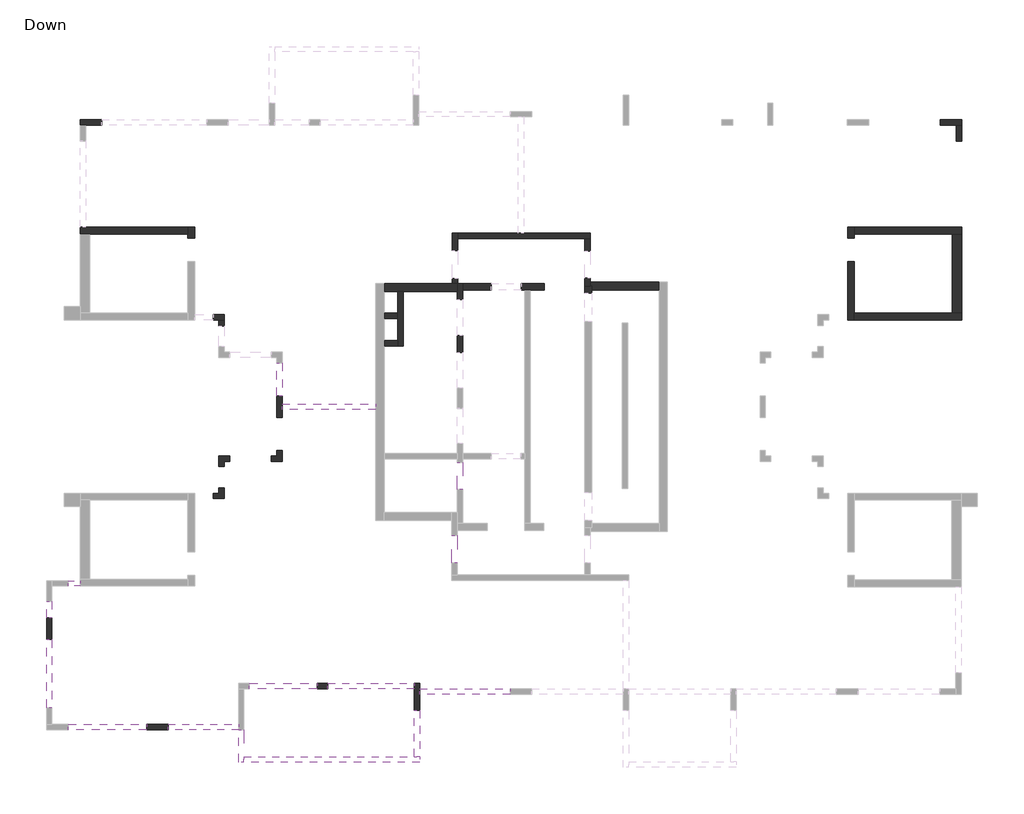
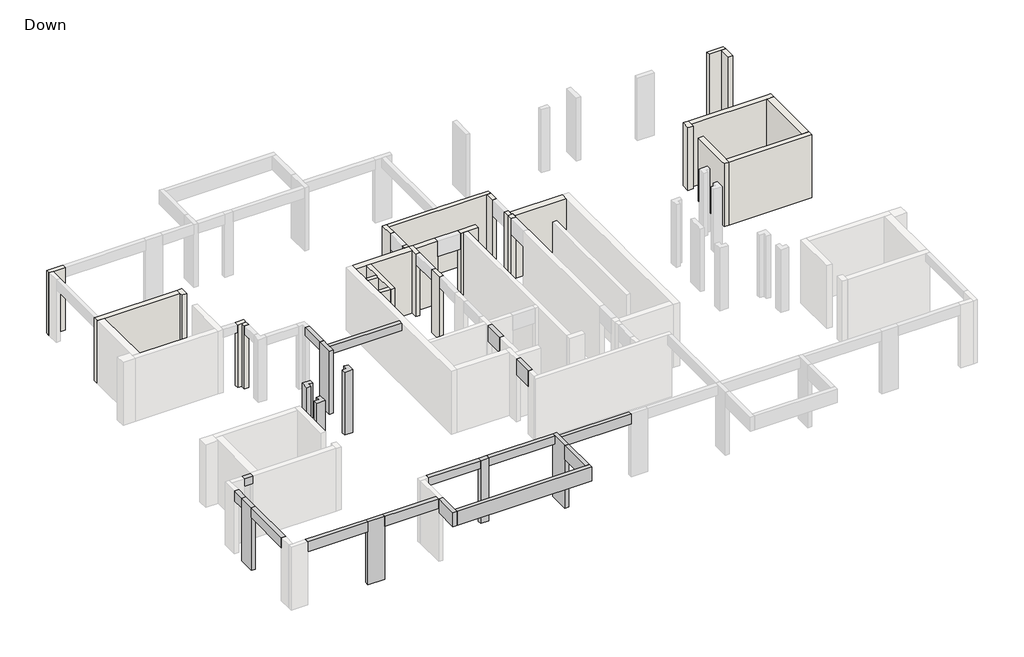
# One storey, part 2 of 3: 27 walls, 15 beams, 8 columns.
"""IFC4 building model written with IfcOpenShell, lengths in millimetres."""

from ifc_helpers import new_model, si_unit, frame, origin, origin_with_axes, place, context, project, spatial, polyline, outline, extrude, faceted_brep, element, save

model = new_model("IFC4")

# Units and contexts
model_context = context("Model", 3, world=origin())
ifc_project = project(units=[si_unit("LENGTHUNIT", "METRE", prefix="MILLI")], contexts=[model_context])

# Site, building, storey
site = spatial("IfcSite", under=ifc_project)
building = spatial("IfcBuilding", under=site)
storey = spatial("IfcBuildingStorey", under=building, Name="Down", Elevation=0.0)

# Beams
placement = place(None, origin())
element("IfcBeam", 1, ObjectType="Concrete Rectengular Beam : 20/40", at=placement, inside=storey, context=model_context, shape_type="Brep", body=[
    faceted_brep([(-8897.9894431, -1293.9530422, 3200.0), (-8697.9894431, -1293.9530422, 3200.0), (-8697.9894431, -74.7215151, 3200.0), (-8897.9894431, -74.7215151, 3200.0), (-8897.9894431, -1293.9530422, 2800.0), (-8897.9894431, -74.7215151, 2800.0), (-8697.9894431, -1293.9530422, 2800.0), (-8697.9894431, -74.7215151, 2800.0), (-8697.9894431, -1293.9530422, 3020.0)], [[[0, 1, 2, 3]], [[4, 0, 3, 5]], [[6, 4, 5, 7]], [[1, 8, 6, 7, 2]], [[1, 0, 4, 6, 8]], [[3, 2, 7, 5]]]),
])
element("IfcBeam", 2, ObjectType="Concrete Rectengular Beam : 20/40", at=placement, inside=storey, context=model_context, shape_type="Brep", body=[
    faceted_brep([(-8697.9894431, -1593.9530422, 3200.0), (-8697.9894431, -1793.9530422, 3200.0), (-5227.8189264, -1793.9530422, 3200.0), (-5227.8189264, -1593.9530422, 3200.0), (-8697.9894431, -1793.9530422, 3020.0), (-8697.9894431, -1793.9530422, 2800.0), (-5227.8189264, -1793.9530422, 2800.0), (-5227.8189264, -1793.9530422, 3020.0), (-8697.9894431, -1593.9530422, 2800.0), (-5227.8189264, -1593.9530422, 2800.0), (-8697.9894431, -1593.9530422, 3020.0), (-5227.8189264, -1593.9530422, 3020.0)], [[[0, 1, 2, 3]], [[1, 4, 5, 6, 7, 2]], [[5, 8, 9, 6]], [[8, 10, 0, 3, 11, 9]], [[1, 0, 10, 8, 5, 4]], [[3, 2, 7, 6, 9, 11]]]),
])
element("IfcBeam", 3, ObjectType="Concrete Rectengular Beam : 20/40", at=placement, inside=storey, context=model_context, shape_type="Brep", body=[
    faceted_brep([(-3819.0362853, -12121.300832, 3200.0), (-3819.0362853, -11921.300832, 3200.0), (-7004.989514, -11921.300832, 3200.0), (-7004.989514, -12121.300832, 3200.0), (-3819.0362853, -11921.300832, 3020.0), (-3819.0362853, -11921.300832, 2800.0), (-7004.989514, -11921.300832, 2800.0), (-7004.989514, -11921.300832, 3020.0), (-3819.0362853, -12121.300832, 2800.0), (-7004.989514, -12121.300832, 2800.0), (-3819.0362853, -12121.300832, 3020.0)], [[[0, 1, 2, 3]], [[2, 1, 4, 5, 6, 7]], [[5, 8, 9, 6]], [[8, 10, 0, 3, 9]], [[1, 0, 10, 8, 5, 4]], [[3, 2, 7, 6, 9]]]),
])
element("IfcBeam", 4, ObjectType="Concrete Rectengular Beam : 20/40", at=placement, inside=storey, context=model_context, shape_type="Brep", body=[
    faceted_brep([(-7404.989514, -12121.300832, 3200.0), (-7404.989514, -11921.300832, 3200.0), (-9913.9547043, -11921.300832, 3200.0), (-9913.9547043, -12121.300832, 3200.0), (-7404.989514, -11921.300832, 3020.0), (-7404.989514, -11921.300832, 2800.0), (-9913.9547043, -11921.300832, 2800.0), (-9913.9547043, -11921.300832, 3020.0), (-7404.989514, -12121.300832, 2800.0), (-9913.9547043, -12121.300832, 2800.0)], [[[0, 1, 2, 3]], [[2, 1, 4, 5, 6, 7]], [[5, 8, 9, 6]], [[3, 9, 8, 0]], [[1, 0, 8, 5, 4]], [[3, 2, 7, 6, 9]]]),
])
element("IfcBeam", 5, ObjectType="Concrete Rectengular Beam : 20/40", at=placement, inside=storey, context=model_context, shape_type="Brep", body=[
    faceted_brep([(-16152.3851738, -8327.5852261, 3200.0), (-16152.3851738, -8127.5852261, 3200.0), (-16589.4316206, -8127.5852261, 3200.0), (-16589.4316206, -8327.5852261, 3200.0), (-16589.4316206, -8327.5852261, 3020.0), (-16589.4316206, -8327.5852261, 2800.0), (-16152.3851738, -8327.5852261, 2800.0), (-16152.3851738, -8327.5852261, 3020.0), (-16152.3851738, -8127.5852261, 2800.0), (-16589.4316206, -8127.5852261, 2800.0)], [[[0, 1, 2, 3]], [[0, 3, 4, 5, 6, 7]], [[8, 6, 5, 9]], [[1, 8, 9, 2]], [[1, 0, 7, 6, 8]], [[3, 2, 9, 5, 4]]]),
])
element("IfcBeam", 6, ObjectType="Concrete Rectengular Beam : 20/50", at=placement, inside=storey, context=model_context, shape_type="Brep", body=[
    faceted_brep([(-270.9686735, -12324.2691374, 3200.0), (-270.9686735, -12124.2691374, 3200.0), (-3619.0362853, -12124.2691374, 3200.0), (-3619.0362853, -12324.2691374, 3200.0), (-270.9686735, -12124.2691374, 3020.0), (-270.9686735, -12124.2691374, 2700.0), (-3619.0362853, -12124.2691374, 2700.0), (-3619.0362853, -12124.2691374, 3020.0), (-270.9686735, -12324.2691374, 2700.0), (-3619.0362853, -12324.2691374, 2700.0)], [[[0, 1, 2, 3]], [[2, 1, 4, 5, 6, 7]], [[5, 8, 9, 6]], [[8, 0, 3, 9]], [[1, 0, 8, 5, 4]], [[3, 2, 7, 6, 9]]]),
])
element("IfcBeam", 7, ObjectType="Concrete Rectengular Beam : 20/50", at=placement, inside=storey, context=model_context, shape_type="Brep", body=[
    faceted_brep([(-12898.304807, -13432.1139628, 3200.0), (-12898.304807, -13632.1139628, 3200.0), (-10303.9547043, -13632.1139628, 3200.0), (-10303.9547043, -13432.1139628, 3200.0), (-12898.304807, -13432.1139628, 2700.0), (-10303.9547043, -13432.1139628, 3020.0), (-10303.9547043, -13432.1139628, 2700.0), (-12898.304807, -13632.1139628, 2700.0), (-10303.9547043, -13632.1139628, 2700.0)], [[[0, 1, 2, 3]], [[4, 0, 3, 5, 6]], [[7, 4, 6, 8]], [[1, 7, 8, 2]], [[1, 0, 4, 7]], [[3, 2, 8, 6, 5]]]),
])
element("IfcBeam", 8, ObjectType="Concrete Rectengular Beam : 20/50", at=placement, inside=storey, context=model_context, shape_type="SweptSolid", body=[
    extrude(outline(polyline([(-13698.304807, -13432.1139628), (-13698.304807, -13632.1139628), (-16594.74029, -13632.1139628), (-16594.74029, -13432.1139628), (-13698.304807, -13432.1139628)])), frame((0.0, 0.0, 2700.0), z_axis=(0.0, 0.0, 1.0), x_axis=(1.0, 0.0, 0.0)), (0.0, 0.0, 1.0), 500.0),
])
element("IfcBeam", 9, ObjectType="Concrete Rectengular Beam : 20/50", at=placement, inside=storey, context=model_context, shape_type="SweptSolid", body=[
    extrude(outline(polyline([(-17394.74029, -10293.6732518), (-17194.74029, -10293.6732518), (-17194.74029, -12822.7787814), (-17394.74029, -12822.7787814), (-17394.74029, -10293.6732518)])), frame((0.0, 0.0, 2700.0), z_axis=(0.0, 0.0, 1.0), x_axis=(1.0, 0.0, 0.0)), (0.0, 0.0, 1.0), 500.0),
])
element("IfcBeam", 10, ObjectType="Concrete Rectengular Beam : 20/50", at=placement, inside=storey, context=model_context, shape_type="SweptSolid", body=[
    extrude(outline(polyline([(-17194.74029, -9493.6732518), (-17394.74029, -9493.6732518), (-17394.74029, -8893.4441313), (-17194.74029, -8893.4441313), (-17194.74029, -9493.6732518)])), frame((0.0, 0.0, 2700.0), z_axis=(0.0, 0.0, 1.0), x_axis=(1.0, 0.0, 0.0)), (0.0, 0.0, 1.0), 500.0),
])
element("IfcBeam", 11, ObjectType="Concrete Rectengular Beam : 20/70", at=placement, inside=storey, context=model_context, shape_type="Brep", body=[
    faceted_brep([(-10103.9547043, -13632.1139628, 3200.0), (-10303.9547043, -13632.1139628, 3200.0), (-10303.9547043, -14832.1139628, 3200.0), (-10103.9547043, -14832.1139628, 3200.0), (-10103.9547043, -14632.1139628, 3200.0), (-10303.9547043, -13632.1139628, 2500.0), (-10303.9547043, -14832.1139628, 2500.0), (-10103.9547043, -14832.1139628, 2500.0), (-10103.9547043, -13632.1139628, 2500.0), (-10103.9547043, -14632.1139628, 2500.0)], [[[0, 1, 2, 3, 4]], [[1, 5, 6, 2]], [[7, 6, 5, 8, 9]], [[8, 0, 4, 3, 7, 9]], [[1, 0, 8, 5]], [[3, 2, 6, 7]]]),
])
element("IfcBeam", 12, ObjectType="Concrete Rectengular Beam : 20/70", at=placement, inside=storey, context=model_context, shape_type="Brep", body=[
    faceted_brep([(-3619.0362853, -14832.1139628, 3200.0), (-3619.0362853, -14632.1139628, 3200.0), (-3819.0362853, -14632.1139628, 3200.0), (-10103.9547043, -14632.1139628, 3200.0), (-10103.9547043, -14832.1139628, 3200.0), (-3619.0362853, -14832.1139628, 2500.0), (-10103.9547043, -14832.1139628, 2500.0), (-3619.0362853, -14632.1139628, 2500.0), (-10103.9547043, -14632.1139628, 2500.0), (-3819.0362853, -14632.1139628, 2500.0), (-10103.9547043, -14632.1139628, 3020.0)], [[[0, 1, 2, 3, 4]], [[5, 0, 4, 6]], [[7, 5, 6, 8, 9]], [[1, 7, 9, 8, 10, 3, 2]], [[4, 3, 10, 8, 6]], [[1, 0, 5, 7]]]),
])
element("IfcBeam", 13, ObjectType="Concrete Rectengular Beam : 20/70", at=placement, inside=storey, context=model_context, shape_type="Brep", body=[
    faceted_brep([(-3619.0362853, -12921.300832, 3200.0), (-3819.0362853, -12921.300832, 3200.0), (-3819.0362853, -14632.1139628, 3200.0), (-3619.0362853, -14632.1139628, 3200.0), (-3619.0362853, -12921.300832, 2500.0), (-3619.0362853, -14632.1139628, 2500.0), (-3819.0362853, -12921.300832, 2500.0), (-3819.0362853, -14632.1139628, 2500.0), (-3819.0362853, -14632.1139628, 3020.0)], [[[0, 1, 2, 3]], [[4, 0, 3, 5]], [[6, 4, 5, 7]], [[1, 6, 7, 8, 2]], [[1, 0, 4, 6]], [[3, 2, 8, 7, 5]]]),
])
element("IfcBeam", 14, ObjectType="Concrete Rectengular Beam : 20/78", at=placement, inside=storey, context=model_context, shape_type="Brep", body=[
    faceted_brep([(-2027.8189264, -3753.9530422, 3200.0), (-2227.8189264, -3753.9530422, 3200.0), (-2227.8189264, -4756.1752209, 3200.0), (-2027.8189264, -4756.1752209, 3200.0), (-2227.8189264, -3753.9530422, 2420.0), (-2227.8189264, -4756.1752209, 2420.0), (-2027.8189264, -3753.9530422, 2420.0), (-2027.8189264, -4756.1752209, 2420.0), (-2027.8189264, -4756.1752209, 3020.0), (-2027.8189264, -3753.9530422, 3020.0)], [[[0, 1, 2, 3]], [[1, 4, 5, 2]], [[4, 6, 7, 5]], [[0, 3, 8, 7, 6, 9]], [[1, 0, 9, 6, 4]], [[3, 2, 5, 7, 8]]]),
])
element("IfcBeam", 15, ObjectType="Concrete Rectengular Beam : 20/78", at=placement, inside=storey, context=model_context, shape_type="Brep", body=[
    faceted_brep([(-2424.4804119, -7466.1752209, 3200.0), (-2224.4804119, -7466.1752209, 3200.0), (-2224.4804119, -6461.1752209, 3200.0), (-2424.4804119, -6461.1752209, 3200.0), (-2224.4804119, -7466.1752209, 2420.0), (-2224.4804119, -6461.1752209, 2420.0), (-2424.4804119, -7466.1752209, 2420.0), (-2424.4804119, -6461.1752209, 2420.0), (-2424.4804119, -6461.1752209, 3020.0), (-2424.4804119, -7466.1752209, 3020.0)], [[[0, 1, 2, 3]], [[1, 4, 5, 2]], [[4, 6, 7, 5]], [[0, 3, 8, 7, 6, 9]], [[1, 0, 9, 6, 4]], [[3, 2, 5, 7, 8]]]),
])

# Columns
element("IfcColumn", 16, ObjectType="Concrete Rectengular Column : 20/100", at=placement, inside=storey, context=model_context, shape_type="Brep", body=[
    faceted_brep([(-3619.0362853, -11921.300832, 0.0), (-3619.0362853, -12921.300832, 0.0), (-3819.0362853, -12921.300832, 0.0), (-3819.0362853, -11921.300832, 0.0), (-3619.0362853, -11921.300832, 3200.0), (-3619.0362853, -12124.2691374, 3200.0), (-3619.0362853, -12921.300832, 3200.0), (-3619.0362853, -11921.300832, 3020.0), (-3819.0362853, -12921.300832, 3200.0), (-3819.0362853, -12121.300832, 3200.0), (-3819.0362853, -11921.300832, 3200.0)], [[[0, 1, 2, 3]], [[4, 5, 6, 1, 0, 7]], [[6, 8, 2, 1]], [[8, 9, 10, 3, 2]], [[10, 4, 7, 0, 3]], [[4, 10, 9, 8, 6, 5]]]),
])
element("IfcColumn", 17, ObjectType="Concrete Rectengular Column : 20/40", at=placement, inside=storey, context=model_context, shape_type="SweptSolid", body=[
    extrude(outline(polyline([(-7404.989514, -11921.300832), (-7004.989514, -11921.300832), (-7004.989514, -12121.300832), (-7404.989514, -12121.300832), (-7404.989514, -11921.300832)])), origin_with_axes(), (0.0, 0.0, 1.0), 3200.0),
])
element("IfcColumn", 18, ObjectType="Concrete Rectengular Column : 20/80", at=placement, inside=storey, context=model_context, shape_type="Brep", body=[
    faceted_brep([(-8697.9894431, -1293.9530422, 0.0), (-8697.9894431, -2093.9530422, 0.0), (-8897.9894431, -2093.9530422, 0.0), (-8897.9894431, -1293.9530422, 0.0), (-8697.9894431, -1293.9530422, 3200.0), (-8697.9894431, -1593.9530422, 3200.0), (-8697.9894431, -1793.9530422, 3200.0), (-8697.9894431, -2093.9530422, 3200.0), (-8697.9894431, -2093.9530422, 2800.0), (-8697.9894431, -1293.9530422, 2800.0), (-8897.9894431, -2093.9530422, 3200.0), (-8897.9894431, -2093.9530422, 2800.0), (-8897.9894431, -1293.9530422, 3200.0), (-8897.9894431, -1293.9530422, 2800.0)], [[[0, 1, 2, 3]], [[4, 5, 6, 7, 8, 1, 0, 9]], [[7, 10, 11, 2, 1, 8]], [[10, 12, 13, 3, 2, 11]], [[12, 4, 9, 0, 3, 13]], [[4, 12, 10, 7, 6, 5]]]),
])
element("IfcColumn", 19, ObjectType="Concrete Rectengular Column : 20/80", at=placement, inside=storey, context=model_context, shape_type="SweptSolid", body=[
    extrude(outline(polyline([(-13698.304807, -13432.1139628), (-12898.304807, -13432.1139628), (-12898.304807, -13632.1139628), (-13698.304807, -13632.1139628), (-13698.304807, -13432.1139628)])), origin_with_axes(), (0.0, 0.0, 1.0), 3200.0),
])
element("IfcColumn", 20, ObjectType="Concrete Rectengular Column : 20/80", at=placement, inside=storey, context=model_context, shape_type="SweptSolid", body=[
    extrude(outline(polyline([(-17194.74029, -9493.6732518), (-17194.74029, -10293.6732518), (-17394.74029, -10293.6732518), (-17394.74029, -9493.6732518), (-17194.74029, -9493.6732518)])), origin_with_axes(), (0.0, 0.0, 1.0), 3200.0),
])
element("IfcColumn", 21, ObjectType="L Column : 40/40/20/20", at=placement, inside=storey, context=model_context, shape_type="Brep", body=[
    faceted_brep([(-8697.9894431, -3713.1845693, 0.0), (-9097.9894431, -3713.1845693, 0.0), (-9097.9894431, -3513.1845693, 0.0), (-8897.9894431, -3513.1845693, 0.0), (-8897.9894431, -3313.1845693, 0.0), (-8697.9894431, -3313.1845693, 0.0), (-8697.9894431, -3713.1845693, 3200.0), (-9097.9894431, -3713.1845693, 3200.0), (-9097.9894431, -3713.1845693, 2800.0), (-8697.9894431, -3713.1845693, 3020.0), (-9097.9894431, -3513.1845693, 3200.0), (-9097.9894431, -3513.1845693, 2800.0), (-8897.9894431, -3513.1845693, 3200.0), (-8897.9894431, -3313.1845693, 3200.0), (-8897.9894431, -3313.1845693, 2800.0), (-8697.9894431, -3313.1845693, 3200.0), (-8697.9894431, -3313.1845693, 2800.0)], [[[0, 1, 2, 3, 4, 5]], [[6, 7, 8, 1, 0, 9]], [[7, 10, 11, 2, 1, 8]], [[10, 12, 3, 2, 11]], [[12, 13, 14, 4, 3]], [[13, 15, 16, 5, 4, 14]], [[15, 6, 9, 0, 5, 16]], [[6, 15, 13, 12, 10, 7]]]),
])
element("IfcColumn", 22, ObjectType="L Column : 40/40/20/20", at=placement, inside=storey, context=model_context, shape_type="Brep", body=[
    faceted_brep([(-11031.2965038, -3513.1845693, 0.0), (-10631.2965038, -3513.1845693, 0.0), (-10631.2965038, -3713.1845693, 0.0), (-10831.2965038, -3713.1845693, 0.0), (-10831.2965038, -3913.1845693, 0.0), (-11031.2965038, -3913.1845693, 0.0), (-11031.2965038, -3513.1845693, 3200.0), (-10631.2965038, -3513.1845693, 3200.0), (-10631.2965038, -3513.1845693, 2800.0), (-10631.2965038, -3713.1845693, 3200.0), (-10631.2965038, -3713.1845693, 2800.0), (-10831.2965038, -3713.1845693, 3200.0), (-10831.2965038, -3713.1845693, 3020.0), (-10831.2965038, -3913.1845693, 3200.0), (-10831.2965038, -3913.1845693, 2800.0), (-11031.2965038, -3913.1845693, 3200.0), (-11031.2965038, -3913.1845693, 2800.0)], [[[0, 1, 2, 3, 4, 5]], [[6, 7, 8, 1, 0]], [[7, 9, 10, 2, 1, 8]], [[9, 11, 12, 3, 2, 10]], [[11, 13, 14, 4, 3, 12]], [[13, 15, 16, 5, 4, 14]], [[15, 6, 0, 5, 16]], [[6, 15, 13, 11, 9, 7]]]),
])
element("IfcColumn", 23, ObjectType="L Column : 40/40/20/20", at=placement, inside=storey, context=model_context, shape_type="Brep", body=[
    faceted_brep([(-10831.2965038, -5093.1845693, 0.0), (-11231.2965038, -5093.1845693, 0.0), (-11231.2965038, -4893.1845693, 0.0), (-11031.2965038, -4893.1845693, 0.0), (-11031.2965038, -4693.1845693, 0.0), (-10831.2965038, -4693.1845693, 0.0), (-10831.2965038, -5093.1845693, 3200.0), (-11231.2965038, -5093.1845693, 3200.0), (-11231.2965038, -5093.1845693, 2800.0), (-10831.2965038, -5093.1845693, 3020.0), (-11231.2965038, -4893.1845693, 3200.0), (-11231.2965038, -4893.1845693, 2800.0), (-11031.2965038, -4893.1845693, 3200.0), (-11031.2965038, -4693.1845693, 3200.0), (-11031.2965038, -4693.1845693, 2800.0), (-10831.2965038, -4693.1845693, 3200.0), (-10831.2965038, -4693.1845693, 2800.0)], [[[0, 1, 2, 3, 4, 5]], [[6, 7, 8, 1, 0, 9]], [[7, 10, 11, 2, 1, 8]], [[10, 12, 3, 2, 11]], [[12, 13, 14, 4, 3]], [[13, 15, 16, 5, 4, 14]], [[15, 6, 9, 0, 5, 16]], [[6, 15, 13, 12, 10, 7]]]),
])

# Walls
element("IfcWall", 24, ObjectType="20", at=placement, inside=storey, context=model_context, shape_type="Brep", body=[
    faceted_brep([(-15359.5625137, 8914.1448811, 0.0), (-16152.3851738, 8914.1448811, 0.0), (-16152.3851738, 8914.1448811, 3200.0), (-15359.5625137, 8914.1448811, 3200.0), (-15359.5625137, 8914.1448811, 2700.0), (-15359.5625137, 8714.1448811, 0.0), (-15359.5625137, 8714.1448811, 2700.0), (-15359.5625137, 8714.1448811, 3200.0), (-15952.3851738, 8714.1448811, 3200.0), (-16152.3851738, 8714.1448811, 3200.0), (-16152.3851738, 8714.1448811, 0.0), (-15952.3851738, 8714.1448811, 0.0)], [[[0, 1, 2, 3, 4]], [[5, 6, 7, 8, 9, 10, 11]], [[1, 0, 5, 11, 10]], [[3, 2, 9, 8, 7]], [[0, 4, 3, 7, 6, 5]], [[2, 1, 10, 9]]]),
])
element("IfcWall", 25, ObjectType="20", at=placement, inside=storey, context=model_context, shape_type="Brep", body=[
    faceted_brep([(-11231.2965038, 1505.2784849, 0.0), (-11031.2965038, 1505.2784849, 0.0), (-10831.2965038, 1505.2784849, 0.0), (-10831.2965038, 1505.2784849, 3200.0), (-11031.2965038, 1505.2784849, 3200.0), (-11231.2965038, 1505.2784849, 3200.0), (-11231.2965038, 1505.2784849, 2800.0), (-11231.2965038, 1705.2784849, 0.0), (-11231.2965038, 1705.2784849, 2800.0), (-11231.2965038, 1705.2784849, 3200.0), (-10831.2965038, 1705.2784849, 3200.0), (-10831.2965038, 1705.2784849, 3020.0), (-10831.2965038, 1705.2784849, 0.0)], [[[0, 1, 2, 3, 4, 5, 6]], [[7, 8, 9, 10, 11, 12]], [[2, 1, 0, 7, 12]], [[5, 4, 3, 10, 9]], [[0, 6, 5, 9, 8, 7]], [[3, 2, 12, 11, 10]]]),
])
element("IfcWall", 26, ObjectType="20", at=placement, inside=storey, context=model_context, shape_type="Brep", body=[
    faceted_brep([(-11031.2965038, 1505.2784849, 0.0), (-11031.2965038, 1285.2784849, 0.0), (-11031.2965038, 1285.2784849, 2800.0), (-11031.2965038, 1285.2784849, 3200.0), (-11031.2965038, 1505.2784849, 3200.0), (-10831.2965038, 1505.2784849, 0.0), (-10831.2965038, 1505.2784849, 3200.0), (-10831.2965038, 1285.2784849, 3200.0), (-10831.2965038, 1285.2784849, 2800.0), (-10831.2965038, 1285.2784849, 0.0)], [[[0, 1, 2, 3, 4]], [[5, 6, 7, 8, 9]], [[1, 0, 5, 9]], [[3, 2, 1, 9, 8, 7]], [[4, 3, 7, 6]], [[0, 4, 6, 5]]]),
])
element("IfcWall", 27, ObjectType="20", at=placement, inside=storey, context=model_context, shape_type="Brep", body=[
    faceted_brep([(-2215.274667, 2858.8247791, 0.0), (-2215.274667, 3043.8247791, 0.0), (-2215.274667, 3043.8247791, 2420.0), (-2215.274667, 3043.8247791, 3200.0), (-2215.274667, 2858.8247791, 3200.0), (-2215.274667, 2858.8247791, 3020.0), (-2415.274667, 2858.8247791, 0.0), (-2415.274667, 2858.8247791, 3020.0), (-2415.274667, 2858.8247791, 3200.0), (-2415.274667, 3043.8247791, 3200.0), (-2415.274667, 3043.8247791, 2420.0), (-2415.274667, 3043.8247791, 0.0), (-2227.8189264, 2858.8247791, 0.0), (-2227.8189264, 2858.8247791, 3200.0)], [[[0, 1, 2, 3, 4, 5]], [[6, 7, 8, 9, 10, 11]], [[1, 0, 12, 6, 11]], [[3, 2, 1, 11, 10, 9]], [[4, 3, 9, 8, 13]], [[0, 5, 4, 13, 8, 7, 6, 12]]]),
])
element("IfcWall", 28, ObjectType="20", at=placement, inside=storey, context=model_context, shape_type="Brep", body=[
    faceted_brep([(-2215.274667, 4069.9784533, 0.0), (-2215.274667, 4509.9784533, 0.0), (-2215.274667, 4709.9784533, 0.0), (-2215.274667, 4709.9784533, 3200.0), (-2215.274667, 4509.9784533, 3200.0), (-2215.274667, 4069.9784533, 3200.0), (-2215.274667, 4069.9784533, 2420.0), (-2415.274667, 4069.9784533, 0.0), (-2415.274667, 4069.9784533, 2420.0), (-2415.274667, 4069.9784533, 3200.0), (-2415.274667, 4709.9784533, 3200.0), (-2415.274667, 4709.9784533, 3020.0), (-2415.274667, 4709.9784533, 0.0)], [[[0, 1, 2, 3, 4, 5, 6]], [[7, 8, 9, 10, 11, 12]], [[2, 1, 0, 7, 12]], [[5, 4, 3, 10, 9]], [[0, 6, 5, 9, 8, 7]], [[3, 2, 12, 11, 10]]]),
])
element("IfcWall", 29, ObjectType="20", at=placement, inside=storey, context=model_context, shape_type="Brep", body=[
    faceted_brep([(-2215.274667, 4509.9784533, 0.0), (2484.725333, 4509.9784533, 0.0), (2684.725333, 4509.9784533, 0.0), (2684.725333, 4509.9784533, 3200.0), (2484.725333, 4509.9784533, 3200.0), (-2215.274667, 4509.9784533, 3200.0), (-2215.274667, 4509.9784533, 3020.0), (-2215.274667, 4709.9784533, 0.0), (-2215.274667, 4709.9784533, 3200.0), (29.0313265, 4709.9784533, 3200.0), (229.0313265, 4709.9784533, 3200.0), (2684.725333, 4709.9784533, 3200.0), (2684.725333, 4709.9784533, 3020.0), (2684.725333, 4709.9784533, 0.0)], [[[0, 1, 2, 3, 4, 5, 6]], [[7, 8, 9, 10, 11, 12, 13]], [[2, 1, 0, 7, 13]], [[5, 4, 3, 11, 10, 9, 8]], [[0, 6, 5, 8, 7]], [[3, 2, 13, 12, 11]]]),
])
element("IfcWall", 30, ObjectType="20", at=placement, inside=storey, context=model_context, shape_type="Brep", body=[
    faceted_brep([(2484.725333, 4509.9784533, 0.0), (2484.725333, 4049.9784533, 0.0), (2484.725333, 4049.9784533, 2420.0), (2484.725333, 4049.9784533, 3200.0), (2484.725333, 4509.9784533, 3200.0), (2484.725333, 4509.9784533, 3020.0), (2684.725333, 4509.9784533, 0.0), (2684.725333, 4509.9784533, 3200.0), (2684.725333, 4049.9784533, 3200.0), (2684.725333, 4049.9784533, 2420.0), (2684.725333, 4049.9784533, 0.0)], [[[0, 1, 2, 3, 4, 5]], [[6, 7, 8, 9, 10]], [[1, 0, 6, 10]], [[3, 2, 1, 10, 9, 8]], [[4, 3, 8, 7]], [[0, 5, 4, 7, 6]]]),
])
element("IfcWall", 31, ObjectType="20", at=placement, inside=storey, context=model_context, shape_type="Brep", body=[
    faceted_brep([(15617.6251666, 8714.1448811, 0.0), (16210.4478267, 8714.1448811, 0.0), (16410.4478267, 8714.1448811, 0.0), (16410.4478267, 8714.1448811, 3200.0), (16210.4478267, 8714.1448811, 3200.0), (15617.6251666, 8714.1448811, 3200.0), (15617.6251666, 8714.1448811, 2700.0), (15617.6251666, 8914.1448811, 0.0), (15617.6251666, 8914.1448811, 2700.0), (15617.6251666, 8914.1448811, 3200.0), (16410.4478267, 8914.1448811, 3200.0), (16410.4478267, 8914.1448811, 0.0)], [[[0, 1, 2, 3, 4, 5, 6]], [[7, 8, 9, 10, 11]], [[2, 1, 0, 7, 11]], [[5, 4, 3, 10, 9]], [[0, 6, 5, 9, 8, 7]], [[3, 2, 11, 10]]]),
])
element("IfcWall", 32, ObjectType="20", at=placement, inside=storey, context=model_context, shape_type="Brep", body=[
    faceted_brep([(16210.4478267, 8714.1448811, 0.0), (16210.4478267, 8125.9123109, 0.0), (16210.4478267, 8125.9123109, 2700.0), (16210.4478267, 8125.9123109, 3200.0), (16210.4478267, 8714.1448811, 3200.0), (16210.4478267, 8714.1448811, 3020.0), (16410.4478267, 8714.1448811, 0.0), (16410.4478267, 8714.1448811, 3200.0), (16410.4478267, 8125.9123109, 3200.0), (16410.4478267, 8125.9123109, 2700.0), (16410.4478267, 8125.9123109, 0.0)], [[[0, 1, 2, 3, 4, 5]], [[6, 7, 8, 9, 10]], [[1, 0, 6, 10]], [[3, 2, 1, 10, 9, 8]], [[4, 3, 8, 7]], [[0, 5, 4, 7, 6]]]),
])
element("IfcWall", 33, ObjectType="20", at=placement, inside=storey, context=model_context, shape_type="Brep", body=[
    faceted_brep([(2684.725333, 2766.2932633, 0.0), (2684.725333, 2916.2932633, 0.0), (2684.725333, 3056.2932633, 0.0), (2684.725333, 3056.2932633, 2420.0), (2684.725333, 3056.2932633, 3200.0), (2684.725333, 2916.2932633, 3200.0), (2684.725333, 2766.2932633, 3200.0), (2484.725333, 2766.2932633, 0.0), (2484.725333, 2766.2932633, 3200.0), (2484.725333, 3056.2932633, 3200.0), (2484.725333, 3056.2932633, 2420.0), (2484.725333, 3056.2932633, 0.0)], [[[0, 1, 2, 3, 4, 5, 6]], [[7, 8, 9, 10, 11]], [[2, 1, 0, 7, 11]], [[4, 3, 2, 11, 10, 9]], [[6, 5, 4, 9, 8]], [[0, 6, 8, 7]]]),
])
element("IfcWall", 34, ObjectType="20", at=placement, inside=storey, context=model_context, shape_type="Brep", body=[
    faceted_brep([(-4422.8189264, 2558.8247791, 0.0), (-4422.8189264, 1760.873998, 0.0), (-4422.8189264, 1560.873998, 0.0), (-4422.8189264, 753.8247791, 0.0), (-4422.8189264, 553.8247791, 0.0), (-4422.8189264, 553.8247791, 3200.0), (-4422.8189264, 753.8247791, 3200.0), (-4422.8189264, 1560.873998, 3200.0), (-4422.8189264, 1760.873998, 3200.0), (-4422.8189264, 2558.8247791, 3200.0), (-4222.8189264, 2558.8247791, 0.0), (-4222.8189264, 2558.8247791, 3200.0), (-4222.8189264, 553.8247791, 3200.0), (-4222.8189264, 553.8247791, 0.0)], [[[0, 1, 2, 3, 4, 5, 6, 7, 8, 9]], [[10, 11, 12, 13]], [[4, 3, 2, 1, 0, 10, 13]], [[9, 8, 7, 6, 5, 12, 11]], [[0, 9, 11, 10]], [[5, 4, 13, 12]]]),
])
element("IfcWall", 35, ObjectType="20", at=placement, inside=storey, context=model_context, shape_type="SweptSolid", body=[
    extrude(outline(polyline([(-4927.8189264, 753.8247791), (-4422.8189264, 753.8247791), (-4422.8189264, 553.8247791), (-4927.8189264, 553.8247791), (-4927.8189264, 753.8247791)])), origin_with_axes(), (0.0, 0.0, 1.0), 3200.0),
])
element("IfcWall", 36, ObjectType="20", at=placement, inside=storey, context=model_context, shape_type="SweptSolid", body=[
    extrude(outline(polyline([(-4927.8189264, 1760.873998), (-4422.8189264, 1760.873998), (-4422.8189264, 1560.873998), (-4927.8189264, 1560.873998), (-4927.8189264, 1760.873998)])), origin_with_axes(), (0.0, 0.0, 1.0), 3200.0),
])
element("IfcWall", 37, ObjectType="20", at=placement, inside=storey, context=model_context, shape_type="Brep", body=[
    faceted_brep([(-2227.8189264, 2858.8247791, 0.0), (-2227.8189264, 2558.8247791, 0.0), (-2227.8189264, 2258.8247791, 0.0), (-2227.8189264, 2258.8247791, 2670.0), (-2227.8189264, 2258.8247791, 3200.0), (-2227.8189264, 2558.8247791, 3200.0), (-2227.8189264, 2858.8247791, 3200.0), (-2027.8189264, 2858.8247791, 0.0), (-2027.8189264, 2858.8247791, 3200.0), (-2027.8189264, 2608.8247791, 3200.0), (-2027.8189264, 2258.8247791, 3200.0), (-2027.8189264, 2258.8247791, 3020.0), (-2027.8189264, 2258.8247791, 2670.0), (-2027.8189264, 2258.8247791, 0.0), (-2027.8189264, 2608.8247791, 0.0), (-2215.274667, 2858.8247791, 0.0), (-2032.8189264, 2258.8247791, 3200.0), (-2215.274667, 2858.8247791, 3200.0)], [[[0, 1, 2, 3, 4, 5, 6]], [[7, 8, 9, 10, 11, 12, 13, 14]], [[2, 1, 0, 15, 7, 14, 13]], [[4, 3, 2, 13, 12, 11, 10, 16]], [[6, 5, 4, 16, 10, 9, 8, 17]], [[0, 6, 17, 8, 7, 15]]]),
])
element("IfcWall", 38, ObjectType="20", at=placement, inside=storey, context=model_context, shape_type="Brep", body=[
    faceted_brep([(-2227.8189264, 933.8247791, 0.0), (-2227.8189264, 313.8247791, 0.0), (-2227.8189264, 313.8247791, 2670.0), (-2227.8189264, 313.8247791, 3200.0), (-2227.8189264, 933.8247791, 3200.0), (-2227.8189264, 933.8247791, 2670.0), (-2027.8189264, 933.8247791, 0.0), (-2027.8189264, 933.8247791, 2670.0), (-2027.8189264, 933.8247791, 3020.0), (-2027.8189264, 933.8247791, 3200.0), (-2027.8189264, 313.8247791, 3200.0), (-2027.8189264, 313.8247791, 3020.0), (-2027.8189264, 313.8247791, 2670.0), (-2027.8189264, 313.8247791, 0.0), (-2032.8189264, 313.8247791, 3200.0), (-2032.8189264, 933.8247791, 3200.0)], [[[0, 1, 2, 3, 4, 5]], [[6, 7, 8, 9, 10, 11, 12, 13]], [[1, 0, 6, 13]], [[3, 2, 1, 13, 12, 11, 10, 14]], [[4, 3, 14, 10, 9, 15]], [[0, 5, 4, 15, 9, 8, 7, 6]]]),
])
element("IfcWall", 39, ObjectType="25", at=placement, inside=storey, context=model_context, shape_type="Brep", body=[
    faceted_brep([(-12179.8186713, 4939.6791417, 0.0), (-16152.3851738, 4939.6791417, 0.0), (-16152.3851738, 4939.6791417, 2700.0), (-16152.3851738, 4939.6791417, 3200.0), (-15952.3851738, 4939.6791417, 3200.0), (-12179.8186713, 4939.6791417, 3200.0), (-12179.8186713, 4689.6791417, 0.0), (-12179.8186713, 4689.6791417, 3020.0), (-12179.8186713, 4689.6791417, 3200.0), (-15802.3851738, 4689.6791417, 3200.0), (-16152.3851738, 4689.6791417, 3200.0), (-16152.3851738, 4689.6791417, 0.0), (-15802.3851738, 4689.6791417, 0.0)], [[[0, 1, 2, 3, 4, 5]], [[6, 7, 8, 9, 10, 11, 12]], [[1, 0, 6, 12, 11]], [[5, 4, 3, 10, 9, 8]], [[0, 5, 8, 7, 6]], [[3, 2, 1, 11, 10]]]),
])
element("IfcWall", 40, ObjectType="25", at=placement, inside=storey, context=model_context, shape_type="Brep", body=[
    faceted_brep([(-12179.8186713, 4939.6791417, 0.0), (-12179.8186713, 4689.6791417, 0.0), (-12179.8186713, 4539.6791417, 0.0), (-12179.8186713, 4539.6791417, 3020.0), (-12179.8186713, 4539.6791417, 3200.0), (-12179.8186713, 4689.6791417, 3200.0), (-12179.8186713, 4939.6791417, 3200.0), (-11929.8186713, 4939.6791417, 0.0), (-11929.8186713, 4939.6791417, 3020.0), (-11929.8186713, 4939.6791417, 3200.0), (-11929.8186713, 4539.6791417, 3200.0), (-11929.8186713, 4539.6791417, 3020.0), (-11929.8186713, 4539.6791417, 0.0)], [[[0, 1, 2, 3, 4, 5, 6]], [[7, 8, 9, 10, 11, 12]], [[2, 1, 0, 7, 12]], [[4, 3, 2, 12, 11, 10]], [[6, 5, 4, 10, 9]], [[0, 6, 9, 8, 7]]]),
])
element("IfcWall", 41, ObjectType="25", at=placement, inside=storey, context=model_context, shape_type="Brep", body=[
    faceted_brep([(-2027.8189264, 2608.8247791, 0.0), (-972.8189264, 2608.8247791, 0.0), (-972.8189264, 2608.8247791, 2420.0), (-972.8189264, 2608.8247791, 3200.0), (-2027.8189264, 2608.8247791, 3200.0), (-2027.8189264, 2608.8247791, 3020.0), (-2027.8189264, 2858.8247791, 0.0), (-2027.8189264, 2858.8247791, 3200.0), (-972.8189264, 2858.8247791, 3200.0), (-972.8189264, 2858.8247791, 2420.0), (-972.8189264, 2858.8247791, 0.0)], [[[0, 1, 2, 3, 4, 5]], [[6, 7, 8, 9, 10]], [[1, 0, 6, 10]], [[3, 2, 1, 10, 9, 8]], [[4, 3, 8, 7]], [[0, 5, 4, 7, 6]]]),
])
element("IfcWall", 42, ObjectType="25", at=placement, inside=storey, context=model_context, shape_type="Brep", body=[
    faceted_brep([(12437.8813243, 4689.6791417, 0.0), (16060.4478267, 4689.6791417, 0.0), (16410.4478267, 4689.6791417, 0.0), (16410.4478267, 4689.6791417, 3200.0), (16060.4478267, 4689.6791417, 3200.0), (12437.8813243, 4689.6791417, 3200.0), (12437.8813243, 4689.6791417, 3020.0), (12437.8813243, 4939.6791417, 0.0), (12437.8813243, 4939.6791417, 3200.0), (16210.4478267, 4939.6791417, 3200.0), (16410.4478267, 4939.6791417, 3200.0), (16410.4478267, 4939.6791417, 2700.0), (16410.4478267, 4939.6791417, 0.0)], [[[0, 1, 2, 3, 4, 5, 6]], [[7, 8, 9, 10, 11, 12]], [[2, 1, 0, 7, 12]], [[5, 4, 3, 10, 9, 8]], [[0, 6, 5, 8, 7]], [[3, 2, 12, 11, 10]]]),
])
element("IfcWall", 43, ObjectType="25", at=placement, inside=storey, context=model_context, shape_type="Brep", body=[
    faceted_brep([(12187.8813243, 4939.6791417, 0.0), (12187.8813243, 4539.6791417, 0.0), (12187.8813243, 4539.6791417, 3020.0), (12187.8813243, 4539.6791417, 3200.0), (12187.8813243, 4939.6791417, 3200.0), (12187.8813243, 4939.6791417, 3020.0), (12437.8813243, 4939.6791417, 0.0), (12437.8813243, 4939.6791417, 3200.0), (12437.8813243, 4689.6791417, 3200.0), (12437.8813243, 4539.6791417, 3200.0), (12437.8813243, 4539.6791417, 3020.0), (12437.8813243, 4539.6791417, 0.0), (12437.8813243, 4689.6791417, 0.0)], [[[0, 1, 2, 3, 4, 5]], [[6, 7, 8, 9, 10, 11, 12]], [[1, 0, 6, 12, 11]], [[3, 2, 1, 11, 10, 9]], [[4, 3, 9, 8, 7]], [[0, 5, 4, 7, 6]]]),
])
element("IfcWall", 44, ObjectType="25", at=placement, inside=storey, context=model_context, shape_type="Brep", body=[
    faceted_brep([(12187.8813243, 3668.3687969, 0.0), (12187.8813243, 1505.2784849, 0.0), (12187.8813243, 1505.2784849, 2800.0), (12187.8813243, 1505.2784849, 3200.0), (12187.8813243, 1705.2784849, 3200.0), (12187.8813243, 3668.3687969, 3200.0), (12187.8813243, 3668.3687969, 3020.0), (12437.8813243, 3668.3687969, 0.0), (12437.8813243, 3668.3687969, 3020.0), (12437.8813243, 3668.3687969, 3200.0), (12437.8813243, 1755.2784849, 3200.0), (12437.8813243, 1505.2784849, 3200.0), (12437.8813243, 1505.2784849, 0.0), (12437.8813243, 1755.2784849, 0.0)], [[[0, 1, 2, 3, 4, 5, 6]], [[7, 8, 9, 10, 11, 12, 13]], [[1, 0, 7, 13, 12]], [[5, 4, 3, 11, 10, 9]], [[0, 6, 5, 9, 8, 7]], [[3, 2, 1, 12, 11]]]),
])
element("IfcWall", 45, ObjectType="25", at=placement, inside=storey, context=model_context, shape_type="Brep", body=[
    faceted_brep([(12437.8813243, 1505.2784849, 0.0), (16410.4478267, 1505.2784849, 0.0), (16410.4478267, 1505.2784849, 3200.0), (12437.8813243, 1505.2784849, 3200.0), (12437.8813243, 1755.2784849, 0.0), (12437.8813243, 1755.2784849, 3020.0), (12437.8813243, 1755.2784849, 3200.0), (16060.4478267, 1755.2784849, 3200.0), (16410.4478267, 1755.2784849, 3200.0), (16410.4478267, 1755.2784849, 0.0), (16060.4478267, 1755.2784849, 0.0)], [[[0, 1, 2, 3]], [[4, 5, 6, 7, 8, 9, 10]], [[1, 0, 4, 10, 9]], [[3, 2, 8, 7, 6]], [[0, 3, 6, 5, 4]], [[2, 1, 9, 8]]]),
])
element("IfcWall", 46, ObjectType="25", at=placement, inside=storey, context=model_context, shape_type="Brep", body=[
    faceted_brep([(2484.725333, 2766.2932633, 0.0), (2484.725333, 2496.2932633, 0.0), (2484.725333, 2496.2932633, 2420.0), (2484.725333, 2496.2932633, 3200.0), (2484.725333, 2766.2932633, 3200.0), (2734.725333, 2766.2932633, 0.0), (2734.725333, 2766.2932633, 3200.0), (2734.725333, 2616.2932633, 3200.0), (2734.725333, 2496.2932633, 3200.0), (2734.725333, 2496.2932633, 2420.0), (2734.725333, 2496.2932633, 0.0), (2734.725333, 2616.2932633, 0.0), (2684.725333, 2766.2932633, 0.0), (2684.725333, 2766.2932633, 3200.0)], [[[0, 1, 2, 3, 4]], [[5, 6, 7, 8, 9, 10, 11]], [[1, 0, 12, 5, 11, 10]], [[3, 2, 1, 10, 9, 8]], [[4, 3, 8, 7, 6, 13]], [[0, 4, 13, 6, 5, 12]]]),
])
element("IfcWall", 47, ObjectType="25", at=placement, inside=storey, context=model_context, shape_type="Brep", body=[
    faceted_brep([(132.1810736, 2608.8247791, 0.0), (272.1810736, 2608.8247791, 0.0), (472.1810736, 2608.8247791, 0.0), (992.1810736, 2608.8247791, 0.0), (992.1810736, 2608.8247791, 3020.0), (992.1810736, 2608.8247791, 3200.0), (472.1810736, 2608.8247791, 3200.0), (272.1810736, 2608.8247791, 3200.0), (132.1810736, 2608.8247791, 3200.0), (132.1810736, 2608.8247791, 2420.0), (132.1810736, 2858.8247791, 0.0), (132.1810736, 2858.8247791, 2420.0), (132.1810736, 2858.8247791, 3200.0), (992.1810736, 2858.8247791, 3200.0), (992.1810736, 2858.8247791, 3020.0), (992.1810736, 2858.8247791, 0.0)], [[[0, 1, 2, 3, 4, 5, 6, 7, 8, 9]], [[10, 11, 12, 13, 14, 15]], [[3, 2, 1, 0, 10, 15]], [[5, 4, 3, 15, 14, 13]], [[8, 7, 6, 5, 13, 12]], [[0, 9, 8, 12, 11, 10]]]),
])
element("IfcWall", 48, ObjectType="30", at=placement, inside=storey, context=model_context, shape_type="Brep", body=[
    faceted_brep([(-4927.8189264, 2558.8247791, 0.0), (-4422.8189264, 2558.8247791, 0.0), (-4222.8189264, 2558.8247791, 0.0), (-2227.8189264, 2558.8247791, 0.0), (-2227.8189264, 2558.8247791, 3200.0), (-4222.8189264, 2558.8247791, 3200.0), (-4422.8189264, 2558.8247791, 3200.0), (-4927.8189264, 2558.8247791, 3200.0), (-4927.8189264, 2858.8247791, 0.0), (-4927.8189264, 2858.8247791, 3200.0), (-2415.274667, 2858.8247791, 3200.0), (-2227.8189264, 2858.8247791, 3200.0), (-2227.8189264, 2858.8247791, 0.0), (-2415.274667, 2858.8247791, 0.0)], [[[0, 1, 2, 3, 4, 5, 6, 7]], [[8, 9, 10, 11, 12, 13]], [[3, 2, 1, 0, 8, 13, 12]], [[7, 6, 5, 4, 11, 10, 9]], [[0, 7, 9, 8]], [[4, 3, 12, 11]]]),
])
element("IfcWall", 49, ObjectType="30", at=placement, inside=storey, context=model_context, shape_type="Brep", body=[
    faceted_brep([(5225.8815794, 2916.2932633, 0.0), (2684.725333, 2916.2932633, 0.0), (2684.725333, 2916.2932633, 3020.0), (2684.725333, 2916.2932633, 3200.0), (5225.8815794, 2916.2932633, 3200.0), (5225.8815794, 2616.2932633, 0.0), (5225.8815794, 2616.2932633, 3020.0), (5225.8815794, 2616.2932633, 3200.0), (2734.725333, 2616.2932633, 3200.0), (2734.725333, 2616.2932633, 3020.0), (2734.725333, 2616.2932633, 0.0), (2734.725333, 2766.2932633, 0.0), (2684.725333, 2766.2932633, 0.0), (2684.725333, 2766.2932633, 3200.0), (2734.725333, 2766.2932633, 3200.0)], [[[0, 1, 2, 3, 4]], [[5, 6, 7, 8, 9, 10]], [[1, 0, 5, 10, 11, 12]], [[4, 3, 13, 14, 8, 7]], [[0, 4, 7, 6, 5]], [[3, 2, 1, 12, 13]], [[12, 11, 14, 13]], [[11, 10, 9, 8, 14]]]),
])
element("IfcWall", 50, ObjectType="35", at=placement, inside=storey, context=model_context, shape_type="Brep", body=[
    faceted_brep([(16410.4478267, 1755.2784849, 0.0), (16410.4478267, 4689.6791417, 0.0), (16410.4478267, 4689.6791417, 3200.0), (16410.4478267, 1755.2784849, 3200.0), (16060.4478267, 1755.2784849, 0.0), (16060.4478267, 1755.2784849, 3020.0), (16060.4478267, 1755.2784849, 3200.0), (16060.4478267, 4689.6791417, 3200.0), (16060.4478267, 4689.6791417, 3020.0), (16060.4478267, 4689.6791417, 0.0)], [[[0, 1, 2, 3]], [[4, 5, 6, 7, 8, 9]], [[1, 0, 4, 9]], [[3, 2, 7, 6]], [[0, 3, 6, 5, 4]], [[2, 1, 9, 8, 7]]]),
])

save(model, "model.ifc")

# Revit data of these elements
# Type "Concrete Rectengular Beam : 20/40"
#   Keynote = "09000"
#   Length [instance default] = 152.4 cm
#   b = 20 cm
#   h = 40 cm
#   Structural Material [instance default] = Concrete
#   Assembly Code = ""
# Type "Concrete Rectengular Beam : 20/50"
#   Length [instance default] = 152.4 cm
#   b = 20 cm
#   h = 50 cm
#   Structural Material [instance default] = Concrete
#   Assembly Code = ""
# Type "Concrete Rectengular Beam : 20/70"
#   Length [instance default] = 152.4 cm
#   b = 20 cm
#   h = 70 cm
#   Structural Material [instance default] = Concrete
#   Assembly Code = ""
# Type "Concrete Rectengular Beam : 20/78"
#   Length [instance default] = 152.4 cm
#   b = 20 cm
#   h = 78 cm
#   Structural Material [instance default] = Concrete
#   Assembly Code = ""
# Type "Concrete Rectengular Column : 20/100"
#   b = 20 cm
#   h = 100 cm
#   Structural Material [instance default] = Concrete
# Type "Concrete Rectengular Column : 20/40"
#   b = 20 cm
#   h = 40 cm
#   Structural Material [instance default] = Concrete
# Type "Concrete Rectengular Column : 20/80"
#   b = 20 cm
#   h = 80 cm
#   Structural Material [instance default] = Concrete
# Type "L Column : 40/40/20/20"
#   Small Length = 20 cm
#   Small Depth = 20 cm
#   Depth = 40 cm
#   Length = 40 cm
#   Centroid Y = 30 cm
#   Centroid X = 10 cm
#   Structural Material [instance default] = Concrete, Cast-in-Place gray
# Type "20"
#   Layers, outside or top first: 20 cm "Concrete" (function 1)
# Type "25"
#   Layers, outside or top first: 25 cm "Concrete" (function 1)
# Type "30"
#   Layers, outside or top first: 30 cm "Concrete" (function 1)
# Type "35"
#   Layers, outside or top first: 35 cm "Concrete" (function 1)
# Element 1 (IfcBeam, "Concrete Rectengular Beam : 20/40")
#   Comments = ""
#   Mark = "B4"
#   SOFiSTiK_AMG_Comments = ""
#   SOFiSTiK_AMG_Scheduled = yes
#   SOFiSTiK_AMG_Adjusted = yes
#   Structural Material = Concrete
#   Phase Created = New Construction
#   Materials on its faces: "Concrete"
# Element 2 (IfcBeam, "Concrete Rectengular Beam : 20/40")
#   Comments = ""
#   Mark = "B5"
#   SOFiSTiK_AMG_Comments = ""
#   SOFiSTiK_AMG_Scheduled = yes
#   SOFiSTiK_AMG_Adjusted = yes
#   Structural Material = Concrete
#   Phase Created = New Construction
#   Materials on its faces: "Concrete"
# Element 3 (IfcBeam, "Concrete Rectengular Beam : 20/40")
#   Comments = ""
#   Mark = "B20"
#   SOFiSTiK_AMG_Comments = ""
#   SOFiSTiK_AMG_Scheduled = yes
#   SOFiSTiK_AMG_Adjusted = yes
#   Structural Material = Concrete
#   Phase Created = New Construction
#   Materials on its faces: "Concrete"
# Element 4 (IfcBeam, "Concrete Rectengular Beam : 20/40")
#   Comments = ""
#   Mark = "B21"
#   SOFiSTiK_AMG_Comments = ""
#   SOFiSTiK_AMG_Scheduled = yes
#   SOFiSTiK_AMG_Adjusted = yes
#   Structural Material = Concrete
#   Phase Created = New Construction
#   Materials on its faces: "Concrete"
# Element 5 (IfcBeam, "Concrete Rectengular Beam : 20/40")
#   Comments = ""
#   Mark = "B22"
#   SOFiSTiK_AMG_Comments = ""
#   SOFiSTiK_AMG_Scheduled = yes
#   SOFiSTiK_AMG_Adjusted = yes
#   Structural Material = Concrete
#   Phase Created = New Construction
#   Materials on its faces: "Concrete"
# Element 6 (IfcBeam, "Concrete Rectengular Beam : 20/50")
#   Comments = ""
#   Mark = "B40"
#   SOFiSTiK_AMG_Comments = ""
#   SOFiSTiK_AMG_Scheduled = yes
#   SOFiSTiK_AMG_Adjusted = yes
#   Structural Material = Concrete
#   Phase Created = New Construction
#   Materials on its faces: "Concrete"
# Element 7 (IfcBeam, "Concrete Rectengular Beam : 20/50")
#   Comments = ""
#   Mark = "B42"
#   SOFiSTiK_AMG_Comments = ""
#   SOFiSTiK_AMG_Scheduled = yes
#   SOFiSTiK_AMG_Adjusted = yes
#   Structural Material = Concrete
#   Phase Created = New Construction
#   Materials on its faces: "Concrete"
# Element 8 (IfcBeam, "Concrete Rectengular Beam : 20/50")
#   Comments = ""
#   Mark = "B43"
#   SOFiSTiK_AMG_Comments = ""
#   SOFiSTiK_AMG_Scheduled = yes
#   SOFiSTiK_AMG_Adjusted = yes
#   Structural Material = Concrete
#   Phase Created = New Construction
#   Materials on its faces: "Concrete"
# Element 9 (IfcBeam, "Concrete Rectengular Beam : 20/50")
#   Comments = ""
#   Mark = "B44"
#   SOFiSTiK_AMG_Comments = ""
#   SOFiSTiK_AMG_Scheduled = yes
#   SOFiSTiK_AMG_Adjusted = yes
#   Structural Material = Concrete
#   Phase Created = New Construction
#   Materials on its faces: "Concrete"
# Element 10 (IfcBeam, "Concrete Rectengular Beam : 20/50")
#   Comments = ""
#   Mark = "B45"
#   SOFiSTiK_AMG_Comments = ""
#   SOFiSTiK_AMG_Scheduled = yes
#   SOFiSTiK_AMG_Adjusted = yes
#   Structural Material = Concrete
#   Phase Created = New Construction
#   Materials on its faces: "Concrete"
# Element 11 (IfcBeam, "Concrete Rectengular Beam : 20/70")
#   Comments = ""
#   Mark = "B55"
#   SOFiSTiK_AMG_Comments = ""
#   SOFiSTiK_AMG_Scheduled = yes
#   SOFiSTiK_AMG_Adjusted = yes
#   Structural Material = Concrete
#   Phase Created = New Construction
#   Materials on its faces: "Concrete"
# Element 12 (IfcBeam, "Concrete Rectengular Beam : 20/70")
#   Comments = ""
#   Mark = "B56"
#   SOFiSTiK_AMG_Comments = ""
#   SOFiSTiK_AMG_Scheduled = yes
#   SOFiSTiK_AMG_Adjusted = yes
#   Structural Material = Concrete
#   Phase Created = New Construction
#   Materials on its faces: "Concrete"
# Element 13 (IfcBeam, "Concrete Rectengular Beam : 20/70")
#   Comments = ""
#   Mark = "B57"
#   SOFiSTiK_AMG_Comments = ""
#   SOFiSTiK_AMG_Scheduled = yes
#   SOFiSTiK_AMG_Adjusted = yes
#   Structural Material = Concrete
#   Phase Created = New Construction
#   Materials on its faces: "Concrete"
# Element 14 (IfcBeam, "Concrete Rectengular Beam : 20/78")
#   Comments = ""
#   Mark = "B64"
#   SOFiSTiK_AMG_Comments = ""
#   SOFiSTiK_AMG_Scheduled = yes
#   SOFiSTiK_AMG_Adjusted = yes
#   Structural Material = Concrete
#   Phase Created = New Construction
#   Materials on its faces: "Concrete"
# Element 15 (IfcBeam, "Concrete Rectengular Beam : 20/78")
#   Comments = ""
#   Mark = "B65"
#   SOFiSTiK_AMG_Comments = ""
#   SOFiSTiK_AMG_Scheduled = yes
#   SOFiSTiK_AMG_Adjusted = yes
#   Structural Material = Concrete
#   Phase Created = New Construction
#   Materials on its faces: "Concrete"
# Element 16 (IfcColumn, "Concrete Rectengular Column : 20/100")
#   Comments = ""
#   Mark = "C1"
#   SOFiSTiK_AMG_Comments = ""
#   SOFiSTiK_AMG_Scheduled = yes
#   SOFiSTiK_AMG_Adjusted = yes
#   Structural Material = Concrete
#   Phase Created = New Construction
#   Materials on its faces: "Concrete"
# Element 17 (IfcColumn, "Concrete Rectengular Column : 20/40")
#   Comments = ""
#   Mark = "C6"
#   SOFiSTiK_AMG_Comments = ""
#   SOFiSTiK_AMG_Scheduled = yes
#   SOFiSTiK_AMG_Adjusted = yes
#   Structural Material = Concrete
#   Phase Created = New Construction
#   Materials on its faces: "Concrete"
# Element 18 (IfcColumn, "Concrete Rectengular Column : 20/80")
#   Comments = ""
#   Mark = "C9"
#   SOFiSTiK_AMG_Comments = ""
#   SOFiSTiK_AMG_Scheduled = yes
#   SOFiSTiK_AMG_Adjusted = yes
#   Structural Material = Concrete
#   Phase Created = New Construction
#   Materials on its faces: "Concrete"
# Element 19 (IfcColumn, "Concrete Rectengular Column : 20/80")
#   Comments = ""
#   Mark = "C18"
#   SOFiSTiK_AMG_Comments = ""
#   SOFiSTiK_AMG_Scheduled = yes
#   SOFiSTiK_AMG_Adjusted = yes
#   Structural Material = Concrete
#   Phase Created = New Construction
#   Materials on its faces: "Concrete"
# Element 20 (IfcColumn, "Concrete Rectengular Column : 20/80")
#   Comments = ""
#   Mark = "C19"
#   SOFiSTiK_AMG_Comments = ""
#   SOFiSTiK_AMG_Scheduled = yes
#   SOFiSTiK_AMG_Adjusted = yes
#   Structural Material = Concrete
#   Phase Created = New Construction
#   Materials on its faces: "Concrete"
# Element 21 (IfcColumn, "L Column : 40/40/20/20")
#   Comments = ""
#   Mark = "C22"
#   SOFiSTiK_AMG_Comments = ""
#   SOFiSTiK_AMG_Scheduled = yes
#   SOFiSTiK_AMG_Adjusted = yes
#   Structural Material = Concrete
#   Phase Created = New Construction
# Element 22 (IfcColumn, "L Column : 40/40/20/20")
#   Comments = ""
#   Mark = "C23"
#   SOFiSTiK_AMG_Comments = ""
#   SOFiSTiK_AMG_Scheduled = yes
#   SOFiSTiK_AMG_Adjusted = yes
#   Structural Material = Concrete
#   Phase Created = New Construction
# Element 23 (IfcColumn, "L Column : 40/40/20/20")
#   Comments = ""
#   Mark = "C24"
#   SOFiSTiK_AMG_Comments = ""
#   SOFiSTiK_AMG_Scheduled = yes
#   SOFiSTiK_AMG_Adjusted = yes
#   Structural Material = Concrete
#   Phase Created = New Construction
# Element 24 (IfcWall, "20")
#   Comments = ""
#   Mark = "W1"
#   SOFiSTiK_EdgeZones = "W1"
#   SOFiSTiK_AMG_Comments = ""
#   Top Offset = 0 cm
#   Base Offset = 0 cm
#   wall height = 320 cm
#   SOFiSTiK_AMG_Scheduled = yes
#   SOFiSTiK_AMG_Adjusted = yes
#   Phase Created = New Construction
#   Base Constraint = Down
#   Top Constraint = Typical Floor
#   Materials on its faces: "Concrete"
# Element 25 (IfcWall, "20")
#   Comments = ""
#   Mark = "W3"
#   SOFiSTiK_EdgeZones = "W3"
#   SOFiSTiK_AMG_Comments = ""
#   Top Offset = 0 cm
#   Base Offset = 0 cm
#   wall height = 320 cm
#   SOFiSTiK_AMG_Scheduled = yes
#   SOFiSTiK_AMG_Adjusted = yes
#   Phase Created = New Construction
#   Base Constraint = Down
#   Top Constraint = Typical Floor
#   Materials on its faces: "Concrete"
# Element 26 (IfcWall, "20")
#   Comments = ""
#   Mark = "W4"
#   SOFiSTiK_EdgeZones = "W4"
#   SOFiSTiK_AMG_Comments = ""
#   Top Offset = 0 cm
#   Base Offset = 0 cm
#   wall height = 320 cm
#   SOFiSTiK_AMG_Scheduled = yes
#   SOFiSTiK_AMG_Adjusted = yes
#   Phase Created = New Construction
#   Base Constraint = Down
#   Top Constraint = Typical Floor
#   Materials on its faces: "Concrete"
# Element 27 (IfcWall, "20")
#   Comments = ""
#   Mark = "W9"
#   SOFiSTiK_EdgeZones = "W9"
#   SOFiSTiK_AMG_Comments = ""
#   Top Offset = 0 cm
#   Base Offset = 0 cm
#   wall height = 320 cm
#   SOFiSTiK_AMG_Scheduled = yes
#   SOFiSTiK_AMG_Adjusted = yes
#   Phase Created = New Construction
#   Base Constraint = Down
#   Top Constraint = Typical Floor
#   Materials on its faces: "Concrete"
# Element 28 (IfcWall, "20")
#   Comments = ""
#   Mark = "W10"
#   SOFiSTiK_EdgeZones = "W10"
#   SOFiSTiK_AMG_Comments = ""
#   Top Offset = 0 cm
#   Base Offset = 0 cm
#   wall height = 320 cm
#   SOFiSTiK_AMG_Scheduled = yes
#   SOFiSTiK_AMG_Adjusted = yes
#   Phase Created = New Construction
#   Base Constraint = Down
#   Top Constraint = Typical Floor
#   Materials on its faces: "Concrete"
# Element 29 (IfcWall, "20")
#   Comments = ""
#   Mark = "W11"
#   SOFiSTiK_EdgeZones = "W11"
#   SOFiSTiK_AMG_Comments = ""
#   Top Offset = 0 cm
#   Base Offset = 0 cm
#   wall height = 320 cm
#   SOFiSTiK_AMG_Scheduled = yes
#   SOFiSTiK_AMG_Adjusted = yes
#   Phase Created = New Construction
#   Base Constraint = Down
#   Top Constraint = Typical Floor
#   Materials on its faces: "Concrete"
# Element 30 (IfcWall, "20")
#   Comments = ""
#   Mark = "W12"
#   SOFiSTiK_EdgeZones = "W12"
#   SOFiSTiK_AMG_Comments = ""
#   Top Offset = 0 cm
#   Base Offset = 0 cm
#   wall height = 320 cm
#   SOFiSTiK_AMG_Scheduled = yes
#   SOFiSTiK_AMG_Adjusted = yes
#   Phase Created = New Construction
#   Base Constraint = Down
#   Top Constraint = Typical Floor
#   Materials on its faces: "Concrete"
# Element 31 (IfcWall, "20")
#   Comments = ""
#   Mark = "W13"
#   SOFiSTiK_EdgeZones = "W13"
#   SOFiSTiK_AMG_Comments = ""
#   Top Offset = 0 cm
#   Base Offset = 0 cm
#   wall height = 320 cm
#   SOFiSTiK_AMG_Scheduled = yes
#   SOFiSTiK_AMG_Adjusted = yes
#   Phase Created = New Construction
#   Base Constraint = Down
#   Top Constraint = Typical Floor
#   Materials on its faces: "Concrete"
# Element 32 (IfcWall, "20")
#   Comments = ""
#   Mark = "W14"
#   SOFiSTiK_EdgeZones = "W14"
#   SOFiSTiK_AMG_Comments = ""
#   Top Offset = 0 cm
#   Base Offset = 0 cm
#   wall height = 320 cm
#   SOFiSTiK_AMG_Scheduled = yes
#   SOFiSTiK_AMG_Adjusted = yes
#   Phase Created = New Construction
#   Base Constraint = Down
#   Top Constraint = Typical Floor
#   Materials on its faces: "Concrete"
# Element 33 (IfcWall, "20")
#   Comments = ""
#   Mark = "W21"
#   SOFiSTiK_EdgeZones = "W21"
#   SOFiSTiK_AMG_Comments = ""
#   Top Offset = 0 cm
#   Base Offset = 0 cm
#   wall height = 320 cm
#   SOFiSTiK_AMG_Scheduled = yes
#   SOFiSTiK_AMG_Adjusted = yes
#   Phase Created = New Construction
#   Base Constraint = Down
#   Top Constraint = Typical Floor
#   Materials on its faces: "Concrete"
# Element 34 (IfcWall, "20")
#   Comments = ""
#   Mark = "W22"
#   SOFiSTiK_EdgeZones = "W22"
#   SOFiSTiK_AMG_Comments = ""
#   Top Offset = 0 cm
#   Base Offset = 0 cm
#   wall height = 320 cm
#   SOFiSTiK_AMG_Scheduled = yes
#   SOFiSTiK_AMG_Adjusted = yes
#   Phase Created = New Construction
#   Base Constraint = Down
#   Top Constraint = Typical Floor
#   Materials on its faces: "Concrete"
# Element 35 (IfcWall, "20")
#   Comments = ""
#   Mark = "W23"
#   SOFiSTiK_EdgeZones = "W23"
#   SOFiSTiK_AMG_Comments = ""
#   Top Offset = 0 cm
#   Base Offset = 0 cm
#   wall height = 320 cm
#   SOFiSTiK_AMG_Scheduled = yes
#   SOFiSTiK_AMG_Adjusted = yes
#   Phase Created = New Construction
#   Base Constraint = Down
#   Top Constraint = Typical Floor
#   Materials on its faces: "Concrete"
# Element 36 (IfcWall, "20")
#   Comments = ""
#   Mark = "W24"
#   SOFiSTiK_EdgeZones = "W24"
#   SOFiSTiK_AMG_Comments = ""
#   Top Offset = 0 cm
#   Base Offset = 0 cm
#   wall height = 320 cm
#   SOFiSTiK_AMG_Scheduled = yes
#   SOFiSTiK_AMG_Adjusted = yes
#   Phase Created = New Construction
#   Base Constraint = Down
#   Top Constraint = Typical Floor
#   Materials on its faces: "Concrete"
# Element 37 (IfcWall, "20")
#   Comments = ""
#   Mark = "W25"
#   SOFiSTiK_EdgeZones = "W25"
#   SOFiSTiK_AMG_Comments = ""
#   Top Offset = 0 cm
#   Base Offset = 0 cm
#   wall height = 320 cm
#   SOFiSTiK_AMG_Scheduled = yes
#   SOFiSTiK_AMG_Adjusted = yes
#   Phase Created = New Construction
#   Base Constraint = Down
#   Top Constraint = Typical Floor
#   Materials on its faces: "Concrete"
# Element 38 (IfcWall, "20")
#   Comments = ""
#   Mark = "W26"
#   SOFiSTiK_EdgeZones = "W26"
#   SOFiSTiK_AMG_Comments = ""
#   Top Offset = 0 cm
#   Base Offset = 0 cm
#   wall height = 320 cm
#   SOFiSTiK_AMG_Scheduled = yes
#   SOFiSTiK_AMG_Adjusted = yes
#   Phase Created = New Construction
#   Base Constraint = Down
#   Top Constraint = Typical Floor
#   Materials on its faces: "Concrete"
# Element 39 (IfcWall, "25")
#   Comments = ""
#   Mark = "W60"
#   SOFiSTiK_EdgeZones = "W62"
#   SOFiSTiK_AMG_Comments = ""
#   Top Offset = 0 cm
#   Base Offset = 0 cm
#   wall height = 320 cm
#   SOFiSTiK_AMG_Scheduled = yes
#   SOFiSTiK_AMG_Adjusted = yes
#   Phase Created = New Construction
#   Base Constraint = Down
#   Top Constraint = Typical Floor
#   Materials on its faces: "Concrete"
# Element 40 (IfcWall, "25")
